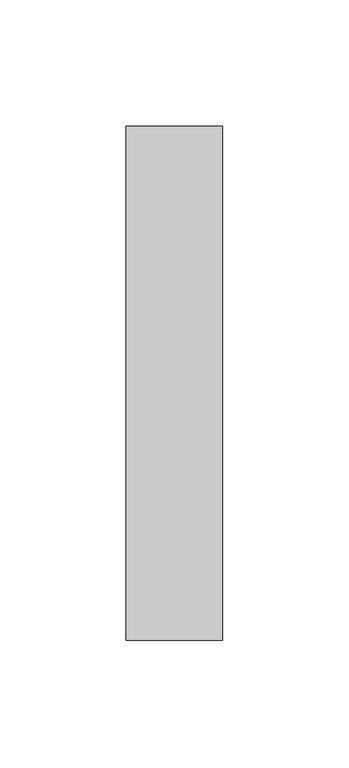
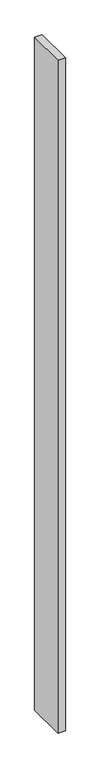
"""IFC4 building model written with IfcOpenShell, lengths in millimetres: proxy geometry, Lower profile:Lower profile:1:Lower profile:1 : Lower profile:Lower profile:300380:301093:Lower profile:1:Lower profile:1 : Lower profile:Lower profile:300380:301093 : Lower profile:Lower profile:1:Lower profile:1 : Lower profile:Lower profile:300380:301093:2 : Lower profile:Lower profile:1:Lower profile:1 : Lower profile:Lower profile:300380:301093:Lower profile:1:Lower profile:1 : Lower profile:Lower profile:300380:301093 : Lower profile:Lower profile:1:Lower profile:1 : Lower profile:Lower profile:300380:301093:300247."""

from ifc_helpers import new_model, si_unit, frame, origin, place, context, project, spatial, polyline, outline, extrude, source, transform, mapped, element, save


def generic_models_94f6f880(model_context):
    return source(origin(), model_context, "Body", "SweptSolid", [
        extrude(outline(polyline([(570490.7367239, -578797.4913841), (570490.7367239, -579000.6913841), (570452.6367239, -579000.6913841), (570452.6367239, -578797.4913841), (570490.7367239, -578797.4913841)])), frame((0.0, 0.0, 25.4), z_axis=(0.0, 0.0, 1.0), x_axis=(1.0, 0.0, 0.0)), (0.0, 0.0, 1.0), 3609.2804687),
    ])


if __name__ == "__main__":
    model = new_model("IFC4")
    model_context = context("Model", 3, world=origin())
    ifc_project = project(units=[si_unit("LENGTHUNIT", "METRE", prefix="MILLI")], contexts=[model_context])
    site = spatial("IfcSite", under=ifc_project)
    building = spatial("IfcBuilding", under=site)
    placement = place(None, origin())
    generic_models_shape = generic_models_94f6f880(model_context)
    element("IfcBuildingElementProxy", 1, Name="Lower profile:Lower profile:1:Lower profile:1 : Lower profile:Lower profile:300380:301093:Lower profile:1:Lower profile:1 : Lower profile:Lower profile:300380:301093 : Lower profile:Lower profile:1:Lower profile:1 : Lower profile:Lower profile:300380:301093:2 : Lower profile:Lower profile:1:Lower profile:1 : Lower profile:Lower profile:300380:301093:Lower profile:1:Lower profile:1 : Lower profile:Lower profile:300380:301093 : Lower profile:Lower profile:1:Lower profile:1 : Lower profile:Lower profile:300380:301093:300247", ObjectType="Lower profile:Lower profile:1:Lower profile:1 : Lower profile:Lower profile:300380:301093:Lower profile:1:Lower profile:1 : Lower profile:Lower profile:300380:301093 : Lower profile:Lower profile:1:Lower profile:1 : Lower profile:Lower profile:300380:301093:2 : Lower profile:Lower profile:1:Lower profile:1 : Lower profile:Lower profile:300380:301093:Lower profile:1:Lower profile:1 : Lower profile:Lower profile:300380:301093 : Lower profile:Lower profile:1:Lower profile:1 : Lower profile:Lower profile:300380:301093:300247", at=placement, inside=building, context=model_context, shape_type="MappedRepresentation", body=[
        mapped(generic_models_shape, transform((0.0, 0.0, 0.0), x_axis=(1.0, 0.0, 0.0), y_axis=(0.0, 1.0, 0.0), z_axis=(0.0, 0.0, 1.0))),
    ])
    save(model, "model.ifc")

# Revit data of these elements
# Type "Lower profile:Lower profile:1:Lower profile:1 : Lower profile:Lower profile:300380:301093:Lower profile:1:Lower profile:1 : Lower profile:Lower profile:300380:301093 : Lower profile:Lower profile:1:Lower profile:1 : Lower profile:Lower profile:300380:301093:2 : Lower profile:Lower profile:1:Lower profile:1 : Lower profile:Lower profile:300380:301093:Lower profile:1:Lower profile:1 : Lower profile:Lower profile:300380:301093 : Lower profile:Lower profile:1:Lower profile:1 : Lower profile:Lower profile:300380:301093:300247"
#   NameOverride = "Lower profile:Lower profile:1:Lower profile:1 : Lower profile:Lower profile:300380:301093:Lower profile:1:Lower profile:1 : Lower profile:Lower profile:300380:301093 : Lower profile:Lower profile:1:Lower profile:1 : Lower profile:Lower profile:300380:301093:300247"
#   ObjectTypeOverride = "Lower profile:1:Lower profile:1 : Lower profile:Lower profile:300380:301093 : Lower profile:Lower profile:1:Lower profile:1 : Lower profile:Lower profile:300380:301093"
#   Reference = "Lower profile"
#   Tag = "300247"
